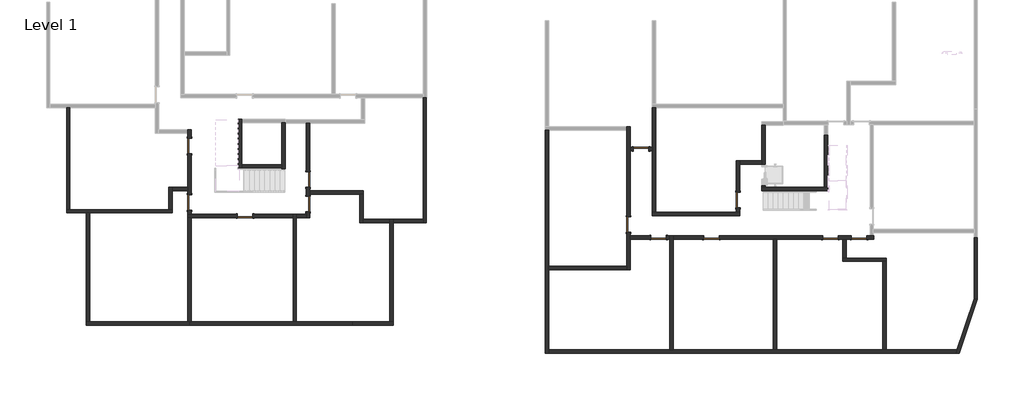
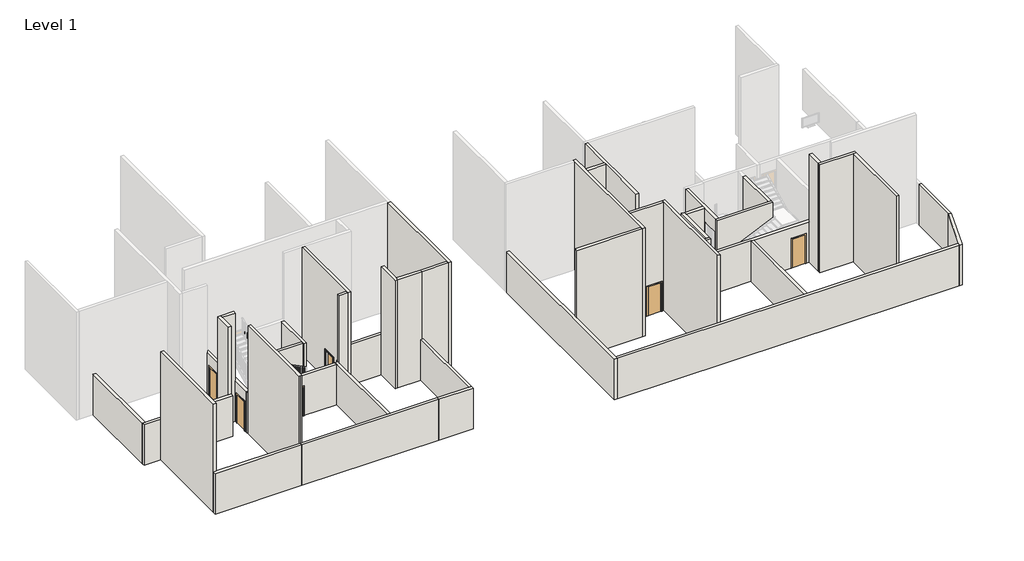
# One storey, part 1 of 3: 44 walls, 12 doors.
# Revit data of these elements (continued)
# Room, not placed, phase "New Construction", upper offset 0 cm, lower offset 0 cm
#   Number = "83"
#   Name = "Room"
# Room, not placed, phase "New Construction", upper offset 0 cm, lower offset 0 cm
#   Number = "84"
#   Name = "5"
# Room, not placed, phase "New Construction", upper offset 0 cm, lower offset 0 cm
#   Number = "85"
#   Name = "Room"
# Room, not placed, phase "New Construction", upper offset 0 cm, lower offset 0 cm
#   Number = "18"
#   Name = "Room"
# Room, not placed, phase "New Construction", upper offset 0 cm, lower offset 0 cm
#   Number = "86"
#   Name = "Room"
# Room, not placed, phase "New Construction", upper offset 0 cm, lower offset 0 cm
#   Number = "137"
#   Name = "Room"
# Room at (15996.482, -9926.883) mm, phase "New Construction", upper level "Level 1", upper offset 243.84 cm, lower offset 0 cm
#   Number = "121"
#   Name = "Room"
# Room at (10068.017, -10568.804) mm, phase "New Construction", upper level "Level 1", upper offset 243.84 cm, lower offset 0 cm
#   Number = "122"
#   Name = "Room"
# Room at (20160.22, -1678.403) mm, phase "New Construction", upper level "Level 1", upper offset 243.84 cm, lower offset 0 cm
#   Number = ""
#   Name = "ASANSÖR"
# Room at (18714.214, -4908.781) mm, phase "New Construction", upper level "Level 1", upper offset 243.84 cm, lower offset 0 cm
#   Number = "49"
#   Name = "Room"
# Room, not placed, phase "New Construction", upper offset 0 cm, lower offset 0 cm
#   Number = "50"
#   Name = "Room"
# Room, not placed, phase "New Construction", upper offset 0 cm, lower offset 0 cm
#   Number = "51"
#   Name = "Room"
# Room, not placed, phase "New Construction", upper offset 0 cm, lower offset 0 cm
#   Number = "52"
#   Name = "Room"
# Room, not placed, phase "New Construction", upper offset 0 cm, lower offset 0 cm
#   Number = "53"
#   Name = "Room"
# Room, not placed, phase "New Construction", upper offset 0 cm, lower offset 0 cm
#   Number = "54"
#   Name = "Room"
# Room, not placed, phase "New Construction", upper offset 0 cm, lower offset 0 cm
#   Number = "55"
#   Name = "Room"
# Room, not placed, phase "New Construction", upper offset 0 cm, lower offset 0 cm
#   Number = "56"
#   Name = "Room"
# Room, not placed, phase "New Construction", upper offset 0 cm, lower offset 0 cm
#   Number = ""
#   Name = "Çamaşır- Kombi"
# Room, not placed, phase "New Construction", upper offset 0 cm, lower offset 0 cm
#   Number = "32"
#   Name = "Room"
# Room, not placed, phase "New Construction", upper offset 0 cm, lower offset 0 cm
#   Number = "33"
#   Name = "Room"
# Room at (7508.93, 3515.695) mm, phase "New Construction", upper level "Level 1", upper offset 243.84 cm, lower offset 0 cm
#   Number = "148"
#   Name = "Room"
# Room at (7233.818, -6185.691) mm, phase "New Construction", upper level "Level 1", upper offset 243.84 cm, lower offset 0 cm
#   Number = "123"
#   Name = "Room"
# Room, not placed, phase "New Construction", upper offset 0 cm, lower offset 0 cm
#   Number = "138"
#   Name = "Room"
# Room at (25542.506, -4072.569) mm, phase "New Construction", upper level "Level 1", upper offset 243.84 cm, lower offset 0 cm
#   Number = "87"
#   Name = "2"
# Room at (21825.305, -10013.945) mm, phase "New Construction", upper level "Level 1", upper offset 243.84 cm, lower offset 0 cm
#   Number = "88"
#   Name = "4"
# Area at (20066.111, 5871.007) mm, upper offset 243.84 cm, lower offset 0 cm
#   Number = "12"
#   Name = "Area"
# Room, not placed, phase "New Construction", upper offset 0 cm, lower offset 0 cm
#   Number = "57"
#   Name = "Room"
# Room, not placed, phase "New Construction", upper offset 0 cm, lower offset 0 cm
#   Number = ""
#   Name = "Room"
# Room, not placed, phase "New Construction", upper offset 0 cm, lower offset 0 cm
#   Number = "59"
#   Name = "Room"
# Room, not placed, phase "New Construction", upper offset 0 cm, lower offset 0 cm
#   Number = "60"
#   Name = "Room"
# Room, not placed, phase "New Construction", upper offset 0 cm, lower offset 0 cm
#   Number = "61"
#   Name = "Room"
# Room, not placed, phase "New Construction", upper offset 0 cm, lower offset 0 cm
#   Number = "62"
#   Name = "Room"
# Room, not placed, phase "New Construction", upper offset 0 cm, lower offset 0 cm
#   Number = "63"
#   Name = "Room"
# Area, not placed, upper offset 0 cm, lower offset 0 cm
#   Number = "5"
#   Name = "Dere Parsel Toplam Alan"
# Room, not placed, phase "New Construction", upper offset 0 cm, lower offset 0 cm
#   Number = "67"
#   Name = "Room"
# Room, not placed, phase "New Construction", upper offset 0 cm, lower offset 0 cm
#   Number = "68"
#   Name = "Room"
# Room at (-14817.024, 11588.139) mm, phase "New Construction", upper level "Level 1", upper offset 243.84 cm, lower offset 0 cm
#   Number = "139"
#   Name = "Room"
# Room at (27717.749, -8269.379) mm, phase "New Construction", upper level "Level 1", upper offset 243.84 cm, lower offset 0 cm
#   Number = "90"
#   Name = "3"
# Area, not placed, upper offset 0 cm, lower offset 0 cm
#   Number = "6"
#   Name = "Area"
# Room, not placed, phase "New Construction", upper offset 0 cm, lower offset 0 cm
#   Number = "93"
#   Name = "6"
# Room, not placed, phase "New Construction", upper offset 0 cm, lower offset 0 cm
#   Number = "5"
#   Name = "Room"
# Room, not placed, phase "New Construction", upper offset 0 cm, lower offset 0 cm
#   Number = "6"
#   Name = "Room"
# Room, not placed, phase "New Construction", upper offset 0 cm, lower offset 0 cm
#   Number = "124"
#   Name = "Room"
# Room at (-20992.701, 5104.389) mm, phase "New Construction", upper level "Level 1", upper offset 243.84 cm, lower offset 0 cm
#   Number = "140"
#   Name = "Room"
# Room at (-18388.177, -2994.154) mm, phase "New Construction", upper level "Level 1", upper offset 243.84 cm, lower offset 0 cm
#   Number = "141"
#   Name = "Room"
# Room, not placed, phase "New Construction", upper offset 0 cm, lower offset 0 cm
#   Number = "34"
#   Name = "Room"
# Room, not placed, phase "New Construction", upper offset 0 cm, lower offset 0 cm
#   Number = "35"
#   Name = "Room"
# Room, not placed, phase "New Construction", upper offset 0 cm, lower offset 0 cm
#   Number = "9"
#   Name = "Room"
# Room, not placed, phase "New Construction", upper offset 0 cm, lower offset 0 cm
#   Number = "10"
#   Name = "Room"
# Room, not placed, phase "New Construction", upper offset 0 cm, lower offset 0 cm
#   Number = "125"
#   Name = "Room"
# Room, not placed, phase "New Construction", upper offset 0 cm, lower offset 0 cm
#   Number = "126"
#   Name = "Room"
# Room, not placed, phase "New Construction", upper offset 0 cm, lower offset 0 cm
#   Number = "127"
#   Name = "Room"
# Room, not placed, phase "New Construction", upper offset 0 cm, lower offset 0 cm
#   Number = "128"
#   Name = "Room"
# Room, not placed, phase "New Construction", upper offset 0 cm, lower offset 0 cm
#   Number = "129"
#   Name = "Room"
# Room, not placed, phase "New Construction", upper offset 0 cm, lower offset 0 cm
#   Number = "91"
#   Name = "Room"
# Room at (-21021.225, 8802.195) mm, phase "New Construction", upper level "Level 1", upper offset 243.84 cm, lower offset 0 cm
#   Number = "130"
#   Name = "Room"
# Room at (-7278.952, -9510.79) mm, phase "New Construction", upper level "Level 1", upper offset 243.84 cm, lower offset 0 cm
#   Number = "131"
#   Name = "Room"
# Room, not placed, phase "New Construction", upper offset 0 cm, lower offset 0 cm
#   Number = "132"
#   Name = "Room"
# Room, not placed, phase "New Construction", upper offset 0 cm, lower offset 0 cm
#   Number = "133"
#   Name = "Room"
# Room, not placed, phase "New Construction", upper offset 0 cm, lower offset 0 cm
#   Number = ""
#   Name = ""
# Room, not placed, phase "New Construction", upper offset 0 cm, lower offset 0 cm
#   Number = "70"
#   Name = "Room"
# Room, not placed, phase "New Construction", upper offset 0 cm, lower offset 0 cm
#   Number = "71"
#   Name = "Room"
# Room, not placed, phase "New Construction", upper offset 0 cm, lower offset 0 cm
#   Number = "92"
#   Name = "Room"
# Room, not placed, phase "New Construction", upper offset 0 cm, lower offset 0 cm
#   Number = ""
#   Name = ""
# Area, not placed, upper offset 0 cm, lower offset 0 cm
#   Number = "10"
#   Name = "Area"
# Area, not placed, upper offset 0 cm, lower offset 0 cm
#   Number = "11"
#   Name = "Area"
# Room, not placed, phase "New Construction", upper offset 0 cm, lower offset 0 cm
#   Number = ""
#   Name = ""
# Room, not placed, phase "New Construction", upper offset 0 cm, lower offset 0 cm
#   Number = "37"
#   Name = "Room"
# Room, not placed, phase "New Construction", upper offset 0 cm, lower offset 0 cm
#   Number = ""
#   Name = "Banyo"
# Room, not placed, phase "New Construction", upper offset 0 cm, lower offset 0 cm
#   Number = ""
#   Name = ""
# Room, not placed, phase "New Construction", upper offset 0 cm, lower offset 0 cm
#   Number = ""
#   Name = "Yatak Odası"
# Room, not placed, phase "New Construction", upper offset 0 cm, lower offset 0 cm
#   Number = "39"
#   Name = "Room"
# Room, not placed, phase "New Construction", upper offset 0 cm, lower offset 0 cm
#   Number = ""
#   Name = "Salon-Mutfak"
# Area, not placed, upper offset 0 cm, lower offset 0 cm
#   Number = "9"
#   Name = "Area"
# Room, not placed, phase "New Construction", upper offset 0 cm, lower offset 0 cm
#   Number = "134"
#   Name = "Room"
# Room, not placed, phase "New Construction", upper offset 0 cm, lower offset 0 cm
#   Number = "135"
#   Name = "Room"
# Room, not placed, phase "New Construction", upper offset 0 cm, lower offset 0 cm
#   Number = "40"
#   Name = "Room"
# Room, not placed, phase "New Construction", upper offset 0 cm, lower offset 0 cm
#   Number = "41"
#   Name = "Room"
# Room at (-12898.035, -7311.307) mm, phase "New Construction", upper level "Level 1", upper offset 243.84 cm, lower offset 0 cm
#   Number = "142"
#   Name = "Room"
# Room, not placed, phase "New Construction", upper offset 0 cm, lower offset 0 cm
#   Number = "143"
#   Name = "Room"
# Room, not placed, phase "New Construction", upper offset 0 cm, lower offset 0 cm
#   Number = "144"
#   Name = "Room"
# Room at (-12608.918, 6284.855) mm, phase "New Construction", upper level "Level 1", upper offset 243.84 cm, lower offset 0 cm
#   Number = "145"
#   Name = "Room"
# Room at (-4085.235, 4670.303) mm, phase "New Construction", upper level "Level 1", upper offset 243.84 cm, lower offset 0 cm
#   Number = "146"
#   Name = "Room"
# Area, not placed, upper offset 0 cm, lower offset 0 cm
#   Number = "8"
#   Name = "Dere Parsel Toplam Alan"
# Room, not placed, phase "New Construction", upper offset 0 cm, lower offset 0 cm
#   Number = "108"
#   Name = "ASANSÖR"
# Room, not placed, phase "New Construction", upper offset 0 cm, lower offset 0 cm
#   Number = "89"
#   Name = "Room"
# Room at (-3408.462, -2181.87) mm, phase "New Construction", upper level "Level 1", upper offset 243.84 cm, lower offset 0 cm
#   Number = "147"
#   Name = "Room"
# Room, not placed, phase "New Construction", upper offset 0 cm, lower offset 0 cm
#   Number = "19"
#   Name = "Room"
# Room, not placed, phase "New Construction", upper offset 0 cm, lower offset 0 cm
#   Number = ""
#   Name = ""
# Room, not placed, phase "New Construction", upper offset 0 cm, lower offset 0 cm
#   Number = "21"
#   Name = "Room"
# Room, not placed, phase "New Construction", upper offset 0 cm, lower offset 0 cm
#   Number = "22"
#   Name = "Room"
# Room, not placed, phase "New Construction", upper offset 0 cm, lower offset 0 cm
#   Number = "23"
#   Name = "Room"
# Room, not placed, phase "New Construction", upper offset 0 cm, lower offset 0 cm
#   Number = "24"
#   Name = "Room"
# Room, not placed, phase "New Construction", upper offset 0 cm, lower offset 0 cm
#   Number = "25"
#   Name = "Room"
# Room, not placed, phase "New Construction", upper offset 0 cm, lower offset 0 cm
#   Number = "64"
#   Name = "Room"
# Room, not placed, phase "New Construction", upper offset 0 cm, lower offset 0 cm
#   Number = "65"
#   Name = "Room"
# Room, not placed, phase "New Construction", upper offset 0 cm, lower offset 0 cm
#   Number = "66"
#   Name = "Room"
# Room, not placed, phase "New Construction", upper offset 0 cm, lower offset 0 cm
#   Number = ""
#   Name = ""
# Room, not placed, phase "New Construction", upper offset 0 cm, lower offset 0 cm
#   Number = "27"
#   Name = "Room"
# Room, not placed, phase "New Construction", upper offset 0 cm, lower offset 0 cm
#   Number = "42"
#   Name = "Room"
# Area, not placed, upper offset 0 cm, lower offset 0 cm
#   Number = "13"
#   Name = "Area"
# Area at (-14699.602, 13833.859) mm, upper offset 243.84 cm, lower offset 0 cm
#   Number = "14"
#   Name = "Area"
# Area, not placed, upper offset 0 cm, lower offset 0 cm
#   Number = "2"
#   Name = "Area"
# Room, not placed, phase "New Construction", upper offset 0 cm, lower offset 0 cm
#   Number = "43"
#   Name = "Room"
# Room, not placed, phase "New Construction", upper offset 0 cm, lower offset 0 cm
#   Number = ""
#   Name = ""
# Room, not placed, phase "New Construction", upper offset 0 cm, lower offset 0 cm
#   Number = "94"
#   Name = "Room"
# Room, not placed, phase "New Construction", upper offset 0 cm, lower offset 0 cm
#   Number = ""
#   Name = ""
# Room, not placed, phase "New Construction", upper offset 0 cm, lower offset 0 cm
#   Number = "136"
#   Name = "Room"
# Room, not placed, phase "New Construction", upper offset 0 cm, lower offset 0 cm
#   Number = "1"
#   Name = "Room"
# Area, not placed, upper offset 0 cm, lower offset 0 cm
#   Number = "3"
#   Name = "Area"
# Room, not placed, phase "New Construction", upper offset 0 cm, lower offset 0 cm
#   Number = "7"
#   Name = "Room"
# Room, not placed, phase "New Construction", upper offset 0 cm, lower offset 0 cm
#   Number = "8"
#   Name = "Room"
# Room, not placed, phase "New Construction", upper offset 0 cm, lower offset 0 cm
#   Number = "2"
#   Name = "Room"
# Room, not placed, phase "New Construction", upper offset 0 cm, lower offset 0 cm
#   Number = "46"
#   Name = "Room"
# Room, not placed, phase "New Construction", upper offset 0 cm, lower offset 0 cm
#   Number = "3"
#   Name = "Room"
# Room, not placed, phase "New Construction", upper offset 0 cm, lower offset 0 cm
#   Number = ""
#   Name = ""
# Room, not placed, phase "New Construction", upper offset 0 cm, lower offset 0 cm
#   Number = "4"
#   Name = "Room"
# Area, not placed, upper offset 0 cm, lower offset 0 cm
#   Number = "1"
#   Name = "Area"
# Room, not placed, phase "New Construction", upper offset 0 cm, lower offset 0 cm
#   Number = ""
#   Name = ""
# Room, not placed, phase "New Construction", upper offset 0 cm, lower offset 0 cm
#   Number = "29"
#   Name = "Room"
# Area, not placed, upper offset 0 cm, lower offset 0 cm
#   Number = "7"
#   Name = "Dere Parsel Toplam Alan"
# Room, not placed, phase "New Construction", upper offset 0 cm, lower offset 0 cm
#   Number = "95"
#   Name = "ASANSÖR"
# Room, not placed, phase "New Construction", upper offset 0 cm, lower offset 0 cm
#   Number = "96"
#   Name = "Room"
# Room, not placed, phase "New Construction", upper offset 0 cm, lower offset 0 cm
#   Number = "97"
#   Name = "7"
# Room, not placed, phase "New Construction", upper offset 0 cm, lower offset 0 cm
#   Number = "98"
#   Name = "8"
# Room, not placed, phase "New Construction", upper offset 0 cm, lower offset 0 cm
#   Number = "99"
#   Name = "9"
# Room, not placed, phase "New Construction", upper offset 0 cm, lower offset 0 cm
#   Number = "100"
#   Name = "1"
# Room, not placed, phase "New Construction", upper offset 0 cm, lower offset 0 cm
#   Number = "101"
#   Name = "5"
# Room, not placed, phase "New Construction", upper offset 0 cm, lower offset 0 cm
#   Number = "102"
#   Name = "2"
# Room, not placed, phase "New Construction", upper offset 0 cm, lower offset 0 cm
#   Number = "103"
#   Name = "4"
# Room, not placed, phase "New Construction", upper offset 0 cm, lower offset 0 cm
#   Number = "104"
#   Name = "3"
# Room, not placed, phase "New Construction", upper offset 0 cm, lower offset 0 cm
#   Number = "105"
#   Name = "6"
